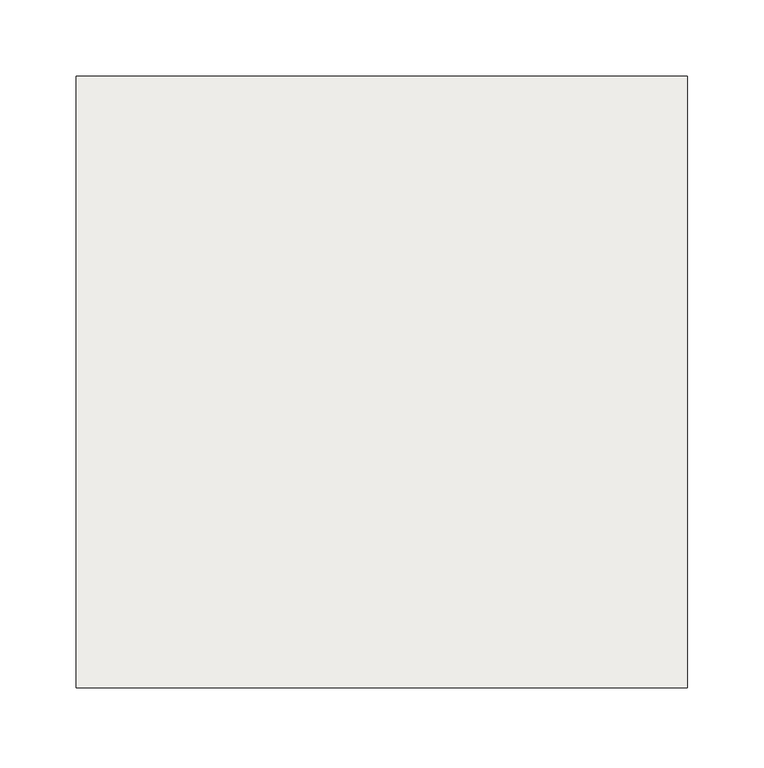
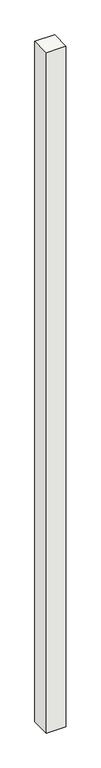
"""IFC4 building model written with IfcOpenShell, lengths in millimetres: slab geometry, NLRS_17_SFO_TLB_funderingspaal geheid beton prefab-AV-MMBPC_gen_rsf : heipaal beton prefab_gen__bxh 400x400."""

from ifc_helpers import new_model, si_unit, frame, origin, place, context, project, spatial, polyline, outline, extrude, source, transform, mapped, element, save


def slab_2462c6b3(model_context):
    return source(origin(), model_context, "Body", "SweptSolid", [
        extrude(outline(polyline([(200.0, -200.0), (-200.0, -200.0), (-200.0, 200.0), (200.0, 200.0), (200.0, -200.0)])), frame((0.0, 0.0, -20000.0), z_axis=(0.0, 0.0, 1.0), x_axis=(1.0, 0.0, 0.0)), (0.0, 0.0, 1.0), 14620.0),
    ])


if __name__ == "__main__":
    model = new_model("IFC4")
    model_context = context("Model", 3, world=origin())
    ifc_project = project(units=[si_unit("LENGTHUNIT", "METRE", prefix="MILLI")], contexts=[model_context])
    site = spatial("IfcSite", under=ifc_project)
    building = spatial("IfcBuilding", under=site)
    placement = place(None, origin())
    slab_shape = slab_2462c6b3(model_context)
    element("IfcSlab", 1, ObjectType="NLRS_17_SFO_TLB_funderingspaal geheid beton prefab-AV-MMBPC_gen_rsf : heipaal beton prefab_gen__bxh 400x400", at=placement, inside=building, context=model_context, shape_type="MappedRepresentation", body=[
        mapped(slab_shape, transform((0.0, 0.0, 0.0), x_axis=(1.0, 0.0, 0.0), y_axis=(0.0, 1.0, 0.0), z_axis=(0.0, 0.0, 1.0))),
    ])
    save(model, "model.ifc")

# Revit data of these elements
# Type "NLRS_17_SFO_TLB_funderingspaal geheid beton prefab-AV-MMBPC_gen_rsf : heipaal beton prefab_gen__bxh 400x400"
#   Export Type to IFC As = "IfcPile"
#   Type IfcGUID = "10$Kfo5uPCAOPJEOo5LE_W"
#   Type Comments = "prefab heipaal 400x400"
#   Model = " "
#   Manufacturer = " "
#   Description = "prefab heipaal 400x400"
#   Assembly Code = "17.21"
#   Width = 400 mm
#   Slanted Angle [instance default] = 0.00°
#   NLRS_S_draagvermogen_trek [instance default] = 0.00 kN
#   NLRS_S_draagvermogen_druk [instance default] = 0.00 kN
#   NLRS_C_lengte [instance default] = 1660 mm
#   NLRS_C_hoogte = 400 mm
#   NLRS_C_breedte = 400 mm
#   Height [instance default] = 1660 mm
#   Length [instance default] = 1660 mm
#   Angle [instance default] = 0.00°
#   Slanted [instance default] = 0
#   Structural Material = NLRS_f2_beton prefab_gen_rsf
#   Keynote = ""
# Element 1 (IfcSlab, "NLRS_17_SFO_TLB_funderingspaal geheid beton prefab-AV-MMBPC_gen_rsf : heipaal beton prefab_gen__bxh 400x400")
#   NLRS_C_lengte = 14620 mm
#   Height = 14620 mm
#   Length = 14620 mm
#   Materials on its faces: "NLRS_f2_beton prefab_gen_rsf"
# Materials
#   "NLRS_f2_beton prefab_gen_rsf": class "F - Niet gebakken kunststeen", colour RGB 129 133 118, transparency 0, Keynote = "f2", Manufacturer = "Revit Standards Foundation", URL = "www.revitstandards.org", Description = "beton prefab", Cost = 0
